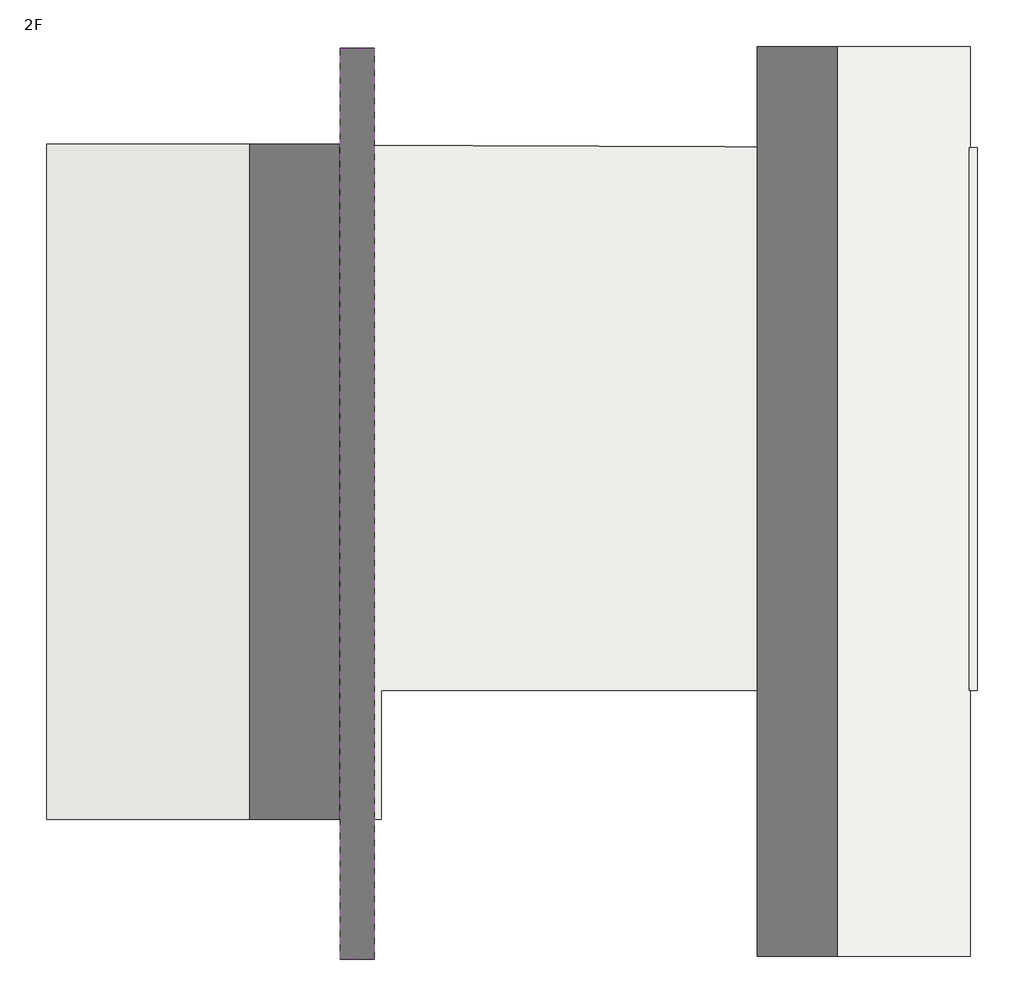
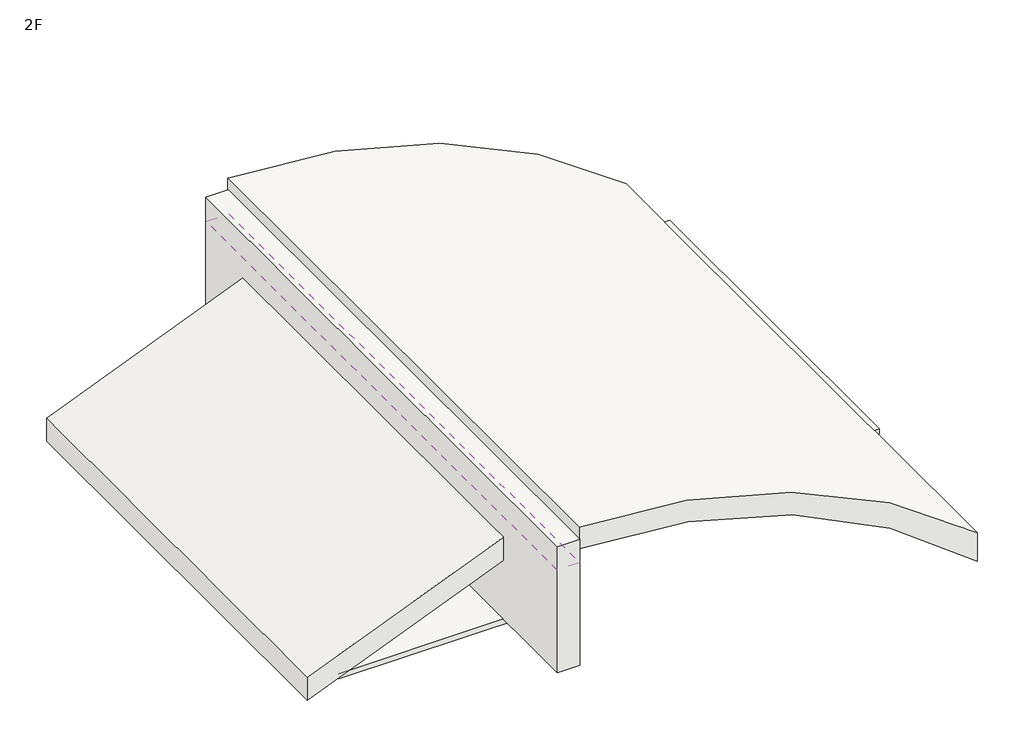
# One storey: 5 roofs.
"""IFC4 building model written with IfcOpenShell, lengths in millimetres."""

from ifc_helpers import new_model, si_unit, point, frame, frame_2d, origin, place, context, project, spatial, polyline, circle_curve, trimmed, segment, composite_curve, outline, extrude, element, save

model = new_model("IFC4")

# Units and contexts
model_context = context("Model", 3, world=origin())
ifc_project = project(units=[si_unit("LENGTHUNIT", "METRE", prefix="MILLI")], contexts=[model_context])

# Site, building, storey
site = spatial("IfcSite", under=ifc_project)
building = spatial("IfcBuilding", under=site)
storey = spatial("IfcBuildingStorey", under=building, Name="2F", Elevation=6450.0)

# Roofs
placement = place(None, origin())
element("IfcRoof", 1, ObjectType="Generic - 400mm", at=placement, inside=storey, context=model_context, shape_type="SweptSolid", body=[
    extrude(outline(composite_curve([segment(polyline([(9109.5004401, -15760.6826666), (8709.4956906, -15760.6826666)]), True, "CONTINUOUS"), segment(trimmed(circle_curve(frame_2d((-1731.4641647, -15708.8367035)), 10441.0885784), [point((8709.4956906, -15760.6826666))], [point((6008.1810273, -8700.6826666))], True, "CARTESIAN"), True, "CONTINUOUS"), segment(polyline([(6008.1810273, -8700.6826666), (6539.8705862, -8700.6826666)]), True, "CONTINUOUS"), segment(trimmed(circle_curve(frame_2d((-1731.4641647, -15708.8367035)), 10841.0885784), [point((6539.8705862, -8700.6826666))], [point((9109.5004401, -15760.6826666))], False, "CARTESIAN"), True, "CONTINUOUS")], self_intersect=False)), frame((0.0, -1718.0210818, 0.0), z_axis=(0.0, 1.0, 0.0), x_axis=(0.0, 0.0, 1.0)), (0.0, 0.0, 1.0), 10780.4577753),
])
element("IfcRoof", 2, ObjectType="Generic - 400mm", at=placement, inside=storey, context=model_context, shape_type="SweptSolid", body=[
    extrude(outline(polyline([(-15760.6826666, -1747.8561761), (-16160.6826666, -1747.8561761), (-16160.6826666, 9042.8723436), (-15760.6826666, 9042.8723436), (-15760.6826666, -1747.8561761)])), frame((0.0, 0.0, 6550.0), z_axis=(0.0, 0.0, 1.0), x_axis=(1.0, 0.0, 0.0)), (0.0, 0.0, 1.0), 2359.4980653),
])
element("IfcRoof", 3, ObjectType="Generic - 400mm", at=placement, inside=storey, context=model_context, shape_type="SweptSolid", body=[
    extrude(outline(polyline([(8909.4980653, -16160.6826666), (8462.2834078, -16160.6826666), (8662.2857825, -15760.6826666), (9109.5004401, -15760.6826666), (8909.4980653, -16160.6826666)])), frame((0.0, -1740.2443602, 0.0), z_axis=(0.0, 1.0, 0.0), x_axis=(0.0, 0.0, 1.0)), (0.0, 0.0, 1.0), 10776.1228455),
])
element("IfcRoof", 4, ObjectType="Generic - 400mm", at=placement, inside=storey, context=model_context, shape_type="SweptSolid", body=[
    extrude(outline(polyline([(6680.6161776, -19639.4433339), (6249.2022805, -19639.4433339), (7672.7073355, -16116.1446865), (8104.1212326, -16116.1446865), (6680.6161776, -19639.4433339)])), frame((0.0, -94.9933886, 0.0), z_axis=(0.0, 1.0, 0.0), x_axis=(0.0, 0.0, 1.0)), (0.0, 0.0, 1.0), 8000.0),
])
element("IfcRoof", 5, ObjectType="roof", at=placement, inside=storey, context=model_context, shape_type="SweptSolid", body=[
    extrude(outline(polyline([(-19076.5903863, -94.9933886), (-19076.5903863, 7905.0066114), (-8616.5903863, 7865.0066114), (-8616.5903863, 1435.0066114), (-15676.5903863, 1435.0066114), (-15676.5903863, -94.9933886), (-19076.5903863, -94.9933886)])), frame((0.0, 0.0, 6450.0), z_axis=(0.0, 0.0, 1.0), x_axis=(1.0, 0.0, 0.0)), (0.0, 0.0, 1.0), 100.0),
])

save(model, "model.ifc")

# Revit data of these elements
# Type "Generic - 400mm"
#   Layers, outside or top first: 40 cm no material (function 1)
# Type "roof"
#   Layers, outside or top first: 10 cm no material (function 1)
# Elements 1, 3 (IfcRoof, "Generic - 400mm")
#   built-in parameter 1001710 = 33615
#   Phase Created = New Construction
#   Materials on its faces: "Default Roof", "Brick, Common"
# Element 2 (IfcRoof, "Generic - 400mm")
#   built-in parameter 1001710 = 33615
#   Phase Created = New Construction
#   Materials on its faces: "Default Roof", "Brick, Common", "Default New Material(1)"
# Element 4 (IfcRoof, "Generic - 400mm")
#   built-in parameter 1001710 = 33615
#   Phase Created = New Construction
#   Materials on its faces: "Default Roof", "Brick, Common", "Parking Stripe"
# Element 5 (IfcRoof, "roof")
#   built-in parameter 1001705 = 21.4895 (stored number, unit not read)
#   built-in parameter 1001710 = 33615
#   Phase Created = New Construction
#   Materials on its faces: "Default Roof", "Earth", "Brick, Common"
# Materials
#   "Default Roof": class "Miscellaneous", colour RGB 0 127 0, transparency 0, Cost = 0
#   "Brick, Common": class "Masonry", colour RGB 170 100 105, transparency 0, Description = "Common brick", Cost = 0
#   "Default New Material(1)": class "Generic", colour RGB 0 255 128, transparency 0, Cost = 0
#   "Parking Stripe": class "Paint", colour RGB 250 250 91, transparency 0, Cost = 0
#   "Earth": class "Generic", colour RGB 97 75 62, transparency 0, Description = "Soil", Cost = 0
